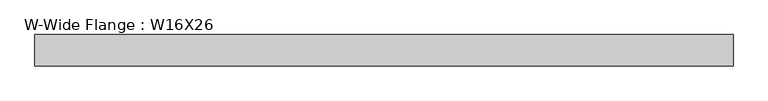
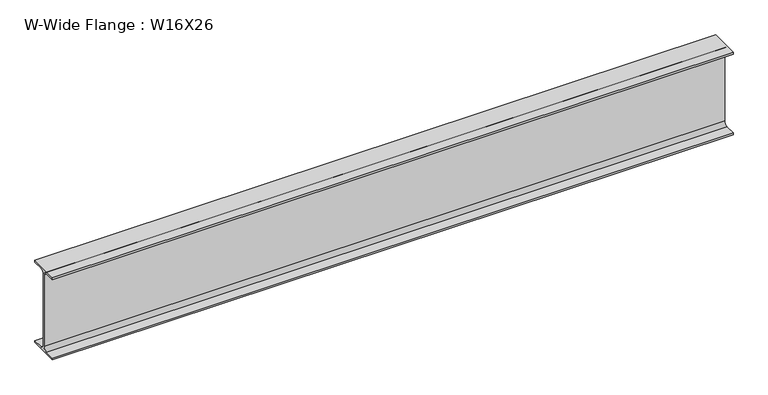
"""IFC4 building model written with IfcOpenShell, lengths in millimetres: beam geometry, W-Wide Flange : W16X26."""

from ifc_helpers import new_model, si_unit, point, frame, frame_2d, origin, place, context, project, spatial, polyline, circle_curve, trimmed, segment, composite_curve, outline, extrude, source, transform, mapped, element, save


def w_wide_flange_w16x26_de54f552(model_context):
    return source(origin(), model_context, "Body", "SweptSolid", [
        extrude(outline(composite_curve([segment(polyline([(69.85, -190.627), (69.85, -199.39), (-69.85, -199.39), (-69.85, -190.627), (-21.3995, -190.627)]), True, "CONTINUOUS"), segment(trimmed(circle_curve(frame_2d((-21.3995, -172.4025)), 18.2245), [point((-21.3995, -190.627))], [point((-3.175, -172.4025))], True, "CARTESIAN"), True, "CONTINUOUS"), segment(polyline([(-3.175, -172.4025), (-3.175, 172.4025)]), True, "CONTINUOUS"), segment(trimmed(circle_curve(frame_2d((-21.3995, 172.4025)), 18.2245), [point((-3.175, 172.4025))], [point((-21.3995, 190.627))], True, "CARTESIAN"), True, "CONTINUOUS"), segment(polyline([(-21.3995, 190.627), (-69.85, 190.627), (-69.85, 199.39), (69.85, 199.39), (69.85, 190.627), (21.3995, 190.627)]), True, "CONTINUOUS"), segment(trimmed(circle_curve(frame_2d((21.3995, 172.4025)), 18.2245), [point((21.3995, 190.627))], [point((3.175, 172.4025))], True, "CARTESIAN"), True, "CONTINUOUS"), segment(polyline([(3.175, 172.4025), (3.175, -172.4025)]), True, "CONTINUOUS"), segment(trimmed(circle_curve(frame_2d((21.3995, -172.4025)), 18.2245), [point((3.175, -172.4025))], [point((21.3995, -190.627))], True, "CARTESIAN"), True, "CONTINUOUS"), segment(polyline([(21.3995, -190.627), (69.85, -190.627)]), True, "CONTINUOUS")], self_intersect=False)), frame((-1650.873, 0.0, 0.0), z_axis=(1.0, 0.0, 0.0), x_axis=(0.0, 1.0, 0.0)), (0.0, 0.0, 1.0), 3124.073),
    ])


if __name__ == "__main__":
    model = new_model("IFC4")
    model_context = context("Model", 3, world=origin())
    ifc_project = project(units=[si_unit("LENGTHUNIT", "METRE", prefix="MILLI")], contexts=[model_context])
    site = spatial("IfcSite", under=ifc_project)
    building = spatial("IfcBuilding", under=site)
    placement = place(None, origin())
    w_wide_flange_w16x26_shape = w_wide_flange_w16x26_de54f552(model_context)
    element("IfcBeam", 1, ObjectType="W-Wide Flange : W16X26", at=placement, inside=building, context=model_context, shape_type="MappedRepresentation", body=[
        mapped(w_wide_flange_w16x26_shape, transform((0.0, 0.0, 0.0), x_axis=(1.0, 0.0, 0.0), y_axis=(0.0, 1.0, 0.0), z_axis=(0.0, 0.0, 1.0))),
    ])
    save(model, "model.ifc")

# Revit data of these elements
# Type "W-Wide Flange : W16X26"
#   Assembly Code = "B10"
#   W = 26
#   Length [instance default] = 5' - 0"
#   bf = 0' - 5 1/2"
#   d = 1' - 3.7"
#   k = 0' - 1 1/16"
#   k2 = 0' - 0.7175"
#   tf = 0' - 0.345"
#   tw = 0' - 0 1/4"
#   A = 0.0533333 SF
#   Structural Material [instance default] = Steel ASTM A992
# Element 1 (IfcBeam, "W-Wide Flange : W16X26")
#   Materials on its faces: "Steel ASTM A992"
# Materials
#   "Steel ASTM A992": class "Metal", colour RGB 199 199 199, transparency 0, Description = "Structural steel 50ksi", Cost = 0
